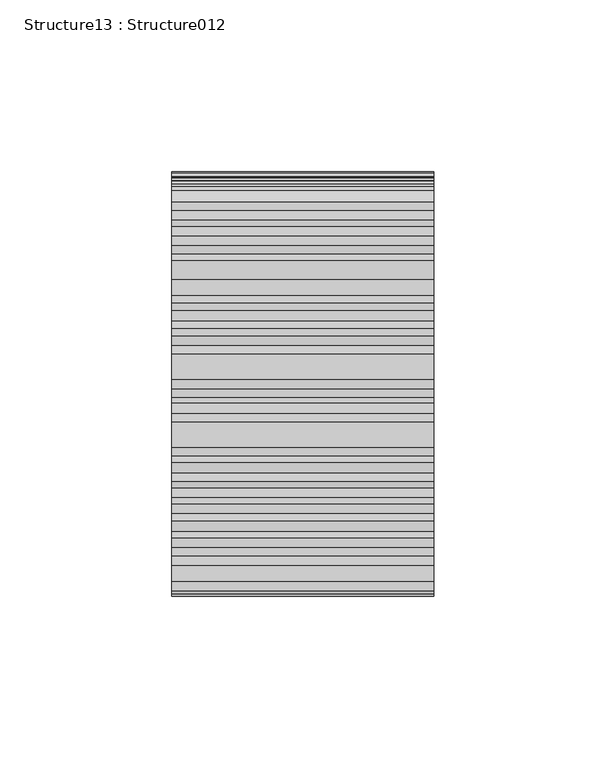
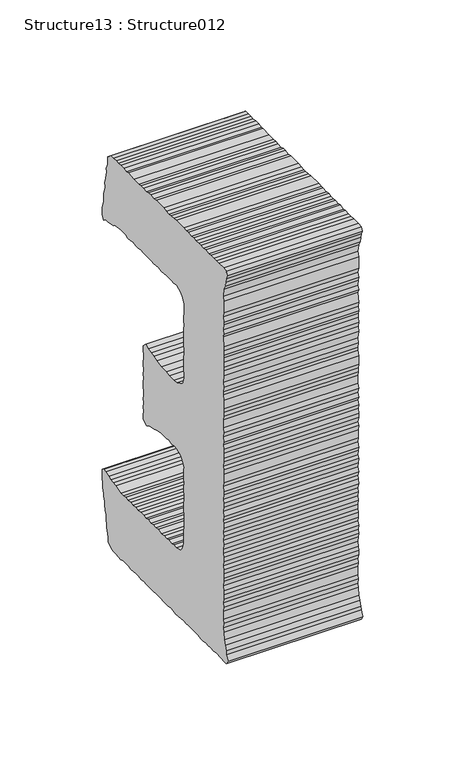
"""IFC4 building model written with IfcOpenShell, lengths in millimetres: proxy geometry, Structure13 : Structure012."""

from ifc_helpers import new_model, si_unit, frame, origin, place, context, project, spatial, polyline, outline, extrude, source, transform, mapped, element, save


def structure13_structure012_19fbd21a(model_context):
    return source(origin(), model_context, "Body", "SweptSolid", [
        extrude(outline(polyline([(3.5276667, 0.0), (5.3743743, -0.6485883), (7.3789606, -2.6086228), (11.6712865, -5.1522585), (12.997503, -6.974613), (17.3925291, -10.3898476), (19.2425048, -11.0356109), (21.500173, -13.1794325), (23.2572465, -14.9471326), (25.2105914, -16.4650146), (27.3033973, -17.2994736), (28.8757889, -19.3131228), (31.027412, -20.5827463), (36.8881158, -25.1369123), (38.155515, -26.5241022), (42.0682255, -29.5645448), (44.6480297, -30.7774346), (46.1678419, -32.3478918), (48.1245316, -33.8683729), (50.1251042, -35.8252884), (51.7863843, -36.713882), (54.1739309, -38.1797088), (55.8837766, -39.5083754), (59.8991872, -43.4204168), (61.8039665, -44.4982258), (63.56104, -46.2659259), (71.1349341, -52.1513576), (73.4712392, -53.175032), (75.4245842, -54.6929141), (76.9963067, -56.7060435), (78.901086, -57.7838524), (80.6621732, -59.5546715), (83.2954431, -61.1985672), (84.8103553, -62.7780916), (88.7230657, -65.8185341), (91.1135054, -67.2737343), (93.0701951, -68.7942154), (92.7742656, -71.6906634), (89.6492424, -73.1966), (88.0787809, -74.7067528), (85.6404446, -76.3396661), (83.380697, -77.7261869), (80.2382233, -80.7678183), (78.4773618, -82.5312788), (77.0174023, -84.9126557), (75.4374391, -86.4433203), (72.3969966, -90.3560306), (71.1262524, -92.4939084), (69.365391, -94.2573688), (68.3369573, -96.584611), (66.6251814, -98.7874758), (65.0599224, -100.3005984), (63.0989293, -102.3216061), (61.6389697, -104.702983), (60.5448162, -106.6122275), (58.7877426, -108.3721942), (57.5132106, -110.5135657), (55.6987344, -111.8448315), (54.4274705, -113.9833781), (52.7214126, -116.1788842), (51.1440485, -117.7062041), (49.6266863, -119.65888), (48.1667268, -122.0402568), (46.4001473, -123.8110759), (45.1262842, -125.9529672), (43.5489202, -127.480287), (42.3291917, -130.0537043), (40.3829028, -132.0571701), (38.9916352, -133.3450045), (37.9637213, -135.6715777), (35.7650962, -137.4972003), (34.4912332, -139.6390916), (33.0311244, -142.0192797), (31.4053438, -143.1077153), (29.9365473, -145.5004643), (28.8595479, -147.3876334), (26.6531255, -149.2232902), (25.3823813, -151.361168), (22.3476568, -155.2665199), (20.8813102, -157.6547354), (19.2529306, -158.7465156), (17.8413876, -161.5667767), (16.518439, -163.269264), (14.5581148, -165.2907915), (13.2861819, -167.4288183), (11.2918471, -168.991542), (10.6298883, -170.8471719), (8.4369812, -172.665436), (7.2146536, -175.2421979), (5.2114818, -176.8162939), (2.1710393, -180.7290042), (1.0858718, -182.6280655), (-0.4288913, -184.5773966), (-1.5142079, -186.4752691), (-4.7485442, -190.6374992), (-6.9383324, -192.4517494), (-8.0725853, -193.9114065), (-9.5408621, -196.3034866), (-11.4961371, -198.3171358), (-13.6666212, -202.1140695), (-15.6123903, -204.1168662), (-16.8921206, -206.2649273), (-18.8389293, -208.269062), (-20.3557718, -210.2210691), (-21.2612297, -211.8874834), (-23.0214222, -213.6514638), (-24.3011524, -215.7995249), (-28.1943993, -219.8059366), (-28.85064, -221.654208), (-30.8512128, -223.2249592), (-32.5050662, -225.8558557), (-33.4048061, -227.5149117), (-35.6034312, -229.3405342), (-36.8205606, -231.9106066), (-40.9999344, -237.2889946), (-43.1892028, -239.102576), (-45.3685238, -242.9108819), (-45.85196, -246.0500109), (-47.3084258, -248.4351756), (-48.3413121, -250.7750513), (-48.9374744, -253.0541027), (-50.9981255, -254.1940738), (-53.395178, -252.7390994), (-57.0576997, -249.8930705), (-59.0630317, -247.9270923), (-61.0150388, -246.4102498), (-63.4087464, -244.9578745), (-64.6775605, -243.5642209), (-67.5075534, -242.1569174), (-68.8324321, -240.3356026), (-71.2268087, -238.8827075), (-72.6924863, -237.7437761), (-74.6944736, -235.780397), (-76.5437803, -235.1351534), (-78.1168409, -233.1209844), (-80.9394753, -231.719399), (-82.2197254, -230.3404623), (-84.3578289, -229.0631053), (-90.2232153, -224.5053005), (-91.9891257, -222.7489727), (-94.2339432, -220.5968979), (-95.4581286, -219.6456225), (-97.6076682, -218.3829824), (-99.9926156, -216.9138109), (-105.8546572, -212.3586053), (-107.4263798, -210.345476), (-110.006853, -209.1320663), (-111.7160298, -207.8039194), (-113.0409086, -205.9826046), (-115.4872724, -204.0816133), (-117.3946506, -203.0071491), (-118.9103086, -201.4216809), (-122.5681476, -198.5792908), (-127.3508164, -195.6546251), (-128.4295202, -194.024605), (-130.76917, -192.9983315), (-132.9693588, -191.2886349), (-134.9787685, -189.3430916), (-136.6312116, -188.4431258), (-138.643966, -186.4949834), (-140.6006557, -184.9745022), (-141.5173264, -181.1132506), (-140.3778752, -179.646904), (-138.860513, -177.6942281), (-137.9381242, -174.4927878), (-136.3671472, -172.9723066), (-135.4679271, -171.3139197), (-134.686857, -168.7955319), (-133.2793278, -165.9721518), (-131.7038172, -164.4541207), (-130.8646756, -162.3649535), (-129.8259945, -160.0231435), (-128.5061648, -158.3246699), (-127.0419018, -155.9294709), (-126.144092, -154.2742795), (-125.1738066, -151.5123926), (-124.080322, -149.6026281), (-122.5634795, -147.6506211), (-119.7689861, -147.0808955), (-119.3079047, -149.0045357), (-117.3068123, -150.9607823), (-115.7261035, -152.9637281), (-113.9638274, -154.7343981), (-113.5039347, -156.6581873), (-109.4835517, -160.5569264), (-105.5708413, -163.597369), (-103.4863526, -164.4425311), (-101.2908465, -166.1485889), (-99.7101377, -168.151535), (-97.3781361, -169.1890315), (-95.6689592, -170.5171783), (-94.0922643, -172.5170053), (-91.4626289, -174.1752432), (-85.6012563, -178.729929), (-83.4565399, -180.0070602), (-81.7473631, -181.3352069), (-79.9271689, -183.5242495), (-77.8420112, -184.3699314), (-75.584343, -186.513753), (-74.3052817, -187.8928388), (-70.3999299, -190.9275632), (-68.2566238, -192.20789), (-66.2443893, -194.1567014), (-62.1231594, -195.4086613), (-59.3210178, -194.8277126), (-56.2114401, -193.3430335), (-52.7962054, -188.9480075), (-51.8969853, -187.2896205), (-50.4408904, -184.9063135), (-48.2337223, -183.0766006), (-47.7778391, -181.4792635), (-46.0058355, -179.7083678), (-44.3018569, -177.5155375), (-42.845762, -175.1322305), (-41.5082584, -173.4110125), (-39.5048607, -171.8435294), (-38.1819121, -170.1410422), (-36.9540923, -167.5503088), (-35.6342627, -165.8518354), (-33.6756428, -163.8407852), (-32.4051246, -161.6962947), (-30.4006873, -160.1274738), (-29.2534388, -158.6510929), (-27.6269125, -154.0409345), (-30.3189996, -148.4342075), (-32.569761, -146.2828783), (-35.9927972, -143.6229459), (-38.8128326, -142.2180158), (-42.724874, -139.178093), (-46.7128765, -137.2603968), (-49.7276279, -136.0936183), (-51.8122658, -135.2472673), (-54.3920701, -134.0343776), (-57.1039128, -133.4870749), (-57.7267376, -130.2500585), (-56.834646, -128.6022256), (-53.3050491, -125.0706943), (-51.6604076, -122.4433684), (-50.7542807, -120.7774737), (-48.7566011, -119.2173491), (-47.1057218, -116.5819958), (-45.7192776, -115.3086525), (-44.4961362, -112.7239398), (-42.7931972, -110.5324473), (-40.7804428, -108.9529231), (-39.2636004, -107.0009161), (-38.1741294, -105.0880327), (-36.606787, -103.5818936), (-35.3930023, -101.009222), (-33.5663444, -99.6691832), (-32.2996139, -97.5281866), (-30.5935561, -95.3326804), (-26.999424, -95.7566219), (-26.0603303, -98.0688764), (-24.7315146, -99.887886), (-22.6542248, -102.2638345), (-21.2774356, -104.5278216), (-18.1846395, -108.1070238), (-16.2798603, -109.1848327), (-14.029768, -111.3356421), (-12.7514479, -112.7184433), (-9.9288136, -114.1200287), (-8.4152392, -115.6985134), (-6.2117056, -117.4108091), (-2.0855034, -118.6494667), (-0.5940581, -118.242), (3.5769987, -116.4019819), (4.235093, -114.5444218), (6.3714921, -112.3045896), (7.8888544, -110.3519137), (9.4686683, -108.8200603), (10.2988238, -106.7410766), (11.8213843, -104.781711), (14.0228344, -102.9593566), (15.5401966, -101.0066807), (16.4368176, -99.3516385), (19.2823267, -95.6897857), (21.2343337, -93.6789615), (25.7916186, -87.8142441), (26.6882396, -86.1592019), (28.1448544, -83.7752259), (31.3739925, -79.6196853), (32.6788216, -75.9247064), (32.8372202, -73.7078169), (29.9353439, -69.8746382), (27.7884034, -68.6086535), (26.7056859, -66.9755143), (23.8830515, -65.573929), (22.799665, -63.94027), (20.6556177, -62.6636587), (18.6447934, -60.7116517), (15.8188142, -59.3074672), (14.2457536, -57.2932981), (12.1050511, -56.0192859), (10.5805561, -54.44519), (8.0047656, -53.2354191), (6.6752043, -51.4104655), (4.7773319, -50.3251489), (2.3828785, -48.8668298), (0.3241575, -46.4752695), (-1.5743839, -45.3894331), (-3.34104, -43.6271613), (-5.4345149, -42.7921826), (-7.4898911, -40.4032214), (-9.3391978, -39.757978), (-10.9122584, -37.7438089), (-12.8682791, -36.2238475), (-17.5403693, -34.1758298), (-19.6836753, -32.895503), (-21.7759614, -32.0603751), (-24.0503345, -31.4581923), (-26.8725258, -30.0505138), (-28.4699395, -29.5892065), (-29.1778649, -27.4737518), (-27.2768735, -25.027388), (-25.7621104, -23.0780569), (-24.1343997, -21.9857567), (-21.9930282, -19.732622), (-19.7384789, -18.3527907), (-18.657845, -16.4512795), (-16.3525059, -15.5003748), (-15.0721067, -13.3528335), (-12.8796427, -11.5406625), (-10.8178028, -10.4005423), (-8.9199304, -7.9581922), (-7.1054543, -6.6269265), (-5.7773074, -4.9177497), (-3.5210539, -3.5274408), (-1.3815358, -1.2835949), (0.0, 0.0), (3.5276667, 0.0)])), frame((-35624.0862846, 275508.1921427, 3985.6060189), z_axis=(1.0, 0.0, 1.3542500454377657e-12), x_axis=(0.0, -0.7896236979923399, -0.6135914076719965)), (0.0, 0.0, 1.0), 76.2),
    ])


if __name__ == "__main__":
    model = new_model("IFC4")
    model_context = context("Model", 3, world=origin())
    ifc_project = project(units=[si_unit("LENGTHUNIT", "METRE", prefix="MILLI")], contexts=[model_context])
    site = spatial("IfcSite", under=ifc_project)
    building = spatial("IfcBuilding", under=site)
    placement = place(None, origin())
    structure13_structure012_shape = structure13_structure012_19fbd21a(model_context)
    element("IfcBuildingElementProxy", 1, Name="Structure13 : Structure012", ObjectType="Structure13 : Structure012", at=placement, inside=building, context=model_context, shape_type="MappedRepresentation", body=[
        mapped(structure13_structure012_shape, transform((0.0, 0.0, 0.0), x_axis=(1.0, 0.0, 0.0), y_axis=(0.0, 1.0, 0.0), z_axis=(0.0, 0.0, 1.0))),
    ])
    save(model, "model.ifc")

# Revit data of these elements
# Type "Structure13 : Structure012"
#   NameOverride = "Structure012"
# Element 1 (IfcBuildingElementProxy, "Structure13 : Structure012")
#   Materials on its faces: "BRUSHED ALUMINUM LETTERING"
# Materials
#   "BRUSHED ALUMINUM LETTERING": class "Unassigned", colour RGB 169 181 186, transparency 0, Cost = 0
